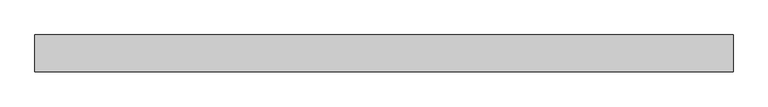
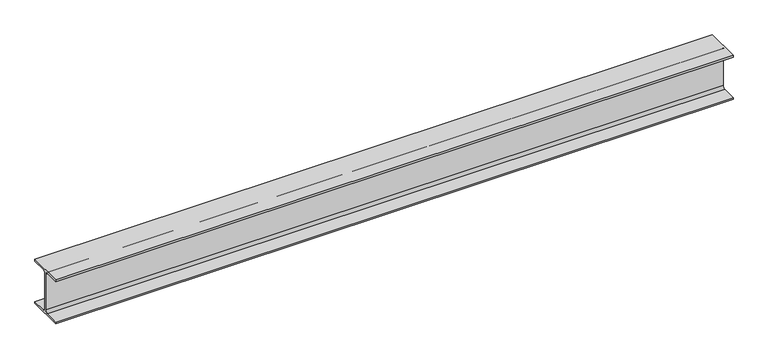
"""IFC4 building model written with IfcOpenShell, lengths in millimetres: beam geometry, 0912_Steel Framing_H-KSD3502 : H_SB_ASB_H-390x300x10x16."""

from ifc_helpers import new_model, si_unit, point, frame, frame_2d, origin, place, context, project, spatial, polyline, circle_curve, trimmed, segment, composite_curve, outline, extrude, source, transform, mapped, element, save


def beam_881ab18f(model_context):
    return source(origin(), model_context, "Body", "SweptSolid", [
        extrude(outline(composite_curve([segment(polyline([(150.0, -179.0), (150.0, -195.0), (-150.0, -195.0), (-150.0, -179.0), (-27.0, -179.0)]), True, "CONTINUOUS"), segment(trimmed(circle_curve(frame_2d((-27.0, -157.0)), 22.0), [point((-27.0, -179.0))], [point((-5.0, -157.0))], True, "CARTESIAN"), True, "CONTINUOUS"), segment(polyline([(-5.0, -157.0), (-5.0, 157.0)]), True, "CONTINUOUS"), segment(trimmed(circle_curve(frame_2d((-27.0, 157.0)), 22.0), [point((-5.0, 157.0))], [point((-27.0, 179.0))], True, "CARTESIAN"), True, "CONTINUOUS"), segment(polyline([(-27.0, 179.0), (-150.0, 179.0), (-150.0, 195.0), (150.0, 195.0), (150.0, 179.0), (27.0, 179.0)]), True, "CONTINUOUS"), segment(trimmed(circle_curve(frame_2d((27.0, 157.0)), 22.0), [point((27.0, 179.0))], [point((5.0, 157.0))], True, "CARTESIAN"), True, "CONTINUOUS"), segment(polyline([(5.0, 157.0), (5.0, -157.0)]), True, "CONTINUOUS"), segment(trimmed(circle_curve(frame_2d((27.0, -157.0)), 22.0), [point((5.0, -157.0))], [point((27.0, -179.0))], True, "CARTESIAN"), True, "CONTINUOUS"), segment(polyline([(27.0, -179.0), (150.0, -179.0)]), True, "CONTINUOUS")], self_intersect=False)), frame((-2837.3, 0.0, 0.0), z_axis=(1.0, 0.0, 0.0), x_axis=(0.0, 1.0, 0.0)), (0.0, 0.0, 1.0), 5674.6),
    ])


if __name__ == "__main__":
    model = new_model("IFC4")
    model_context = context("Model", 3, world=origin())
    ifc_project = project(units=[si_unit("LENGTHUNIT", "METRE", prefix="MILLI")], contexts=[model_context])
    site = spatial("IfcSite", under=ifc_project)
    building = spatial("IfcBuilding", under=site)
    placement = place(None, origin())
    beam_shape = beam_881ab18f(model_context)
    element("IfcBeam", 1, ObjectType="0912_Steel Framing_H-KSD3502 : H_SB_ASB_H-390x300x10x16", at=placement, inside=building, context=model_context, shape_type="MappedRepresentation", body=[
        mapped(beam_shape, transform((0.0, 0.0, 0.0), x_axis=(1.0, 0.0, 0.0), y_axis=(0.0, 1.0, 0.0), z_axis=(0.0, 0.0, 1.0))),
    ])
    save(model, "model.ifc")

# Revit data of these elements
# Type "0912_Steel Framing_H-KSD3502 : H_SB_ASB_H-390x300x10x16"
#   H_WM Code_1 = "S01AA001-00001 | Main Steel Structure Fabrication Work | Shelter/Building | Heavy Steel - Standard (Weight≥90KG/M) | Material: (   )"
#   H_WM Code_2 = "S03AA027-00001 | Main Steel Structure Erection Work | Shelter/Building | Heavy Steel (Weight≥90KG/M) | Material: (   )"
#   H_WM Code_3 = "S01AA010-00001 | Main Steel Structure Fabrication Work | Shelter/Building | Steel Painting/Coating | for Non-Fireproofed Steel Surface, Surface Preparation, Primer, Second & Final Coat | Material: (   )"
#   H_Q'ty Cal Type Tag = "SB-Q2"
#   Width = 30.0 cm
#   Web Thickness = 1.0 cm
#   Web Fillet = 2.2 cm
#   Warping Constant = 2520000.0 cm⁶
#   W = 0
#   Torsional Moment of Inertia = 94.3867 cm⁴
#   Section Area = 136.0 cm²
#   Plastic Modulus weak axis = 733.0 cm³
#   Plastic Modulus strong axis = 2190.0 cm³
#   Perimeter = 1.92 m²/m
#   Nominal Weight = 107.00 kgf/m
#   Moment of Inertia weak axis = 7210.00 cm⁴
#   Moment of Inertia strong axis = 38700.00 cm⁴
#   Height = 39.0 cm
#   Flange Thickness = 1.6 cm
#   Elastic Modulus weak axis = 481.0 cm³
#   Elastic Modulus strong axis = 1980.0 cm³
#   Centroid Vertical = 19.5 cm
#   Centroid Horizontal = 15.0 cm
#   Ix = 387000000
#   Length [instance default] = 1.5240 m
#   Zx = 2190000
#   b = 0.3000 m
#   h = 0.3900 m
#   r = 0.0220 m
#   s = 0.0100 m
#   t = 0.0160 m
#   A = 0.0136 m²
#   Structural Material [instance default] = Steel, 45-345
#   Assembly Code = ""
# Element 1 (IfcBeam, "0912_Steel Framing_H-KSD3502 : H_SB_ASB_H-390x300x10x16")
#   Structural Material = none
# Materials
#   "Steel, 45-345": class "Metal", colour RGB 189 187 185, transparency 0, Description = "Steel 345 MPa", Cost = 0
